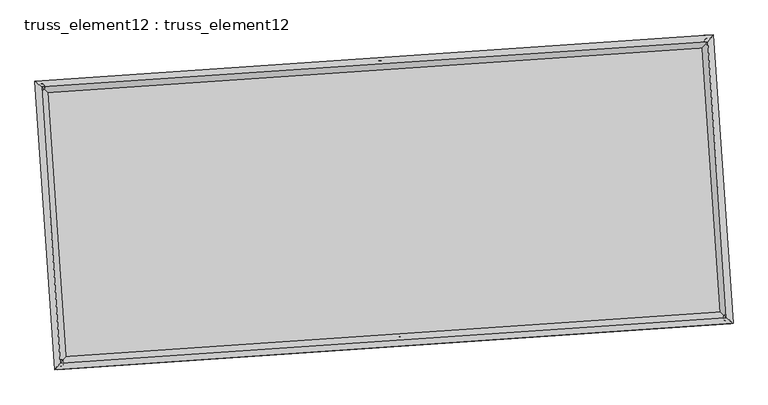
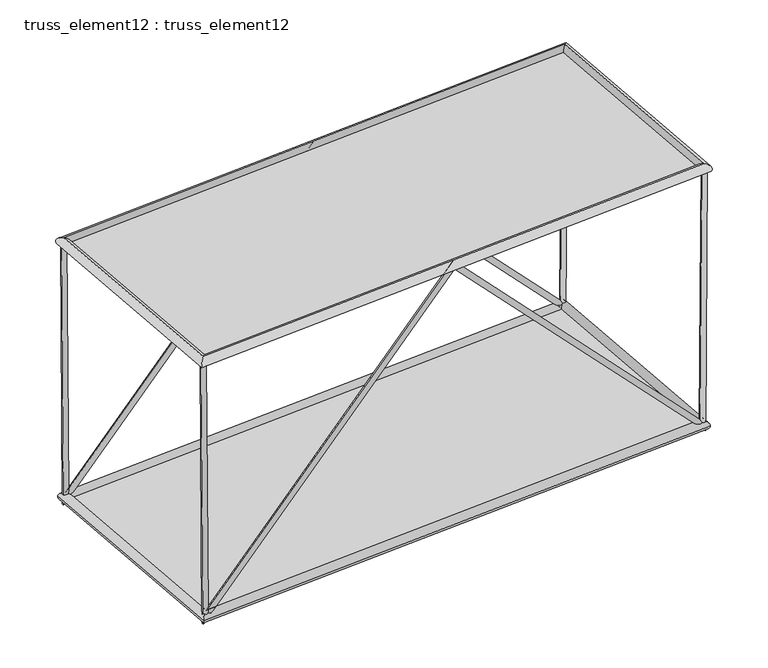
"""IFC4 building model written with IfcOpenShell, lengths in millimetres: plate geometry, truss_element12 : truss_element12."""

from ifc_helpers import new_model, si_unit, frame, origin, origin_with_axes, place, context, project, spatial, polyline, circle_curve, ellipse_curve, outline, extrude, source, transform, mapped, element, save
from ifc_brep_helpers import plane_surface, cylinder_surface, advanced_brep


def truss_element12_truss_element12_8b6da639(model_context):
    return source(origin(), model_context, "Body", "SolidModel", [
        advanced_brep(
        [(-3700.3653821, 2273.8085663, 5000.2282154), (-3799.4662365, 2260.4474806, 4999.5196659), (-3665.8139539, 2276.1644968, 123.2875786), (-3763.1729289, 2262.9221833, -123.2875786), (1064.0023703, 2598.6726923, 5071.9949185), (1064.4463477, 2592.0991902, 4927.7489333), (5793.2665802, 2921.1432411, 123.2835929), (5891.4943968, 2921.2372474, -123.2835929), (5828.3659378, 2923.5365329, 5000.2298034), (5928.3631169, 2923.7511852, 4999.5100189)],
        [
            (0, 1, circle_curve(frame((-3749.9158093, 2267.1280234, 4999.8739406), z_axis=(-0.007084473580338079, -0.0004830633228379881, 0.9999747881241386), x_axis=(-0.13361091131504388, 0.9910337559845098, -0.00046784270723809073)), 50.0)),
            (1, 0, circle_curve(frame((-3749.9158093, 2267.1280234, 4999.8739406), z_axis=(-0.007084473580338079, -0.0004830633228379881, 0.9999747881241386), x_axis=(-0.13361091131504388, 0.9910337559845098, -0.00046784270723809073)), 50.0)),
            (0, 2),
            (2, 3, ellipse_curve(frame((-3714.4934414, 2269.54334, 0.0), z_axis=(-0.9270962013206413, -0.06321516574545871, 0.3694542953013412), x_axis=(0.3685984160306923, 0.025133324815376896, 0.9292489029766943)), 132.9633385, 50.0)),
            (3, 1),
            (3, 2, ellipse_curve(frame((-3714.4934414, 2269.54334, 0.0), z_axis=(-0.9270962013206413, -0.06321516574545871, 0.3694542953013412), x_axis=(0.3685984160306923, 0.025133324815376896, 0.9292489029766943)), 132.9633385, 50.0)),
            (2, 4),
            (4, 5, ellipse_curve(frame((1064.224359, 2595.3859413, 4999.8719259), z_axis=(-0.9976833956449117, -0.06802823819938442, 2.935858576566568e-05), x_axis=(-2.929057355045047e-05, -1.9972128665769184e-06, -0.9999999995690367)), 72.2800399, 50.0)),
            (5, 3),
            (5, 4, ellipse_curve(frame((1064.224359, 2595.3859413, 4999.8719259), z_axis=(-0.9976833956449117, -0.06802823819938442, 2.935858576566568e-05), x_axis=(-2.929057355045047e-05, -1.9972128665769184e-06, -0.9999999995690367)), 72.2800399, 50.0)),
            (4, 6),
            (6, 7, ellipse_curve(frame((5842.3804885, 2921.1902443, 0.0), z_axis=(-0.9271277711546797, -0.0632173183724334, -0.3693746967667848), x_axis=(-0.3685190018944136, -0.02512790986730541, 0.9292805461153513)), 132.9545126, 50.0)),
            (7, 5),
            (7, 6, ellipse_curve(frame((5842.3804885, 2921.1902443, 0.0), z_axis=(-0.9271277711546797, -0.0632173183724334, -0.3693746967667848), x_axis=(-0.3685190018944136, -0.02512790986730541, 0.9292805461153513)), 132.9545126, 50.0)),
            (8, 9, circle_curve(frame((5878.3645274, 2923.6438591, 4999.8699112), z_axis=(0.007196807775672843, 0.0004907229645955706, 0.9999739822359441), x_axis=(-0.002149999800475158, 0.9999975758109794, -0.00047526100493728435)), 50.0)),
            (9, 8, circle_curve(frame((5878.3645274, 2923.6438591, 4999.8699112), z_axis=(0.007196807775672843, 0.0004907229645955706, 0.9999739822359441), x_axis=(-0.002149999800475158, 0.9999975758109794, -0.00047526100493728435)), 50.0)),
            (6, 8),
            (9, 7),
        ],
        [
            plane_surface(frame((-3749.9158093, 2317.1280176, 4999.8980944), z_axis=(-0.0070844735803373745, -0.00048306332284137114, 0.9999747881241386), x_axis=(0.9999749048021603, -3.422335232095009e-06, 0.007084472753714267))),
            cylinder_surface(frame((-3749.9158093, 2267.1280234, 4999.8739406), z_axis=(-0.007084473580338079, -0.0004830633228379881, 0.9999747881241386), x_axis=(-0.13361091131504388, 0.9910337559845098, -0.00046784270723809073)), 50.0),
            cylinder_surface(frame((-3714.4934414, 2269.54334, 0.0), z_axis=(-0.690172538563737, -0.0470602418132238, -0.7221130109982568), x_axis=(-0.020414395916308354, 0.9987521960693102, -0.04557744273324799)), 50.0),
            cylinder_surface(frame((1064.224359, 2595.3859413, 4999.8719259), z_axis=(-0.6901302351654778, -0.04705735730530667, 0.7221536288310701), x_axis=(-0.1153491321235071, 0.9922789572880589, -0.04557464911193756)), 50.0),
            plane_surface(frame((5878.3645274, 2873.6438651, 4999.894448), z_axis=(0.007196807775673034, 0.0004907229645977637, 0.999973982235944), x_axis=(0.9999741026435836, -3.531730309092038e-06, -0.007196806909099957))),
            cylinder_surface(frame((5842.3804885, 2921.1902443, 0.0), z_axis=(-0.007196807775672843, -0.0004907229645955706, -0.9999739822359441), x_axis=(-0.002149999800475158, 0.9999975758109794, -0.00047526100493728435)), 50.0),
        ],
        [
            (0, [[1, 2]]),
            (1, [[-1, 3, 4, 5]]),
            (1, [[-2, -5, 6, -3]]),
            (2, [[-4, 7, 8, 9]]),
            (2, [[-6, -9, 10, -7]]),
            (3, [[-8, 11, 12, 13]]),
            (3, [[-10, -13, 14, -11]]),
            (4, [[15, 16]]),
            (5, [[-12, 17, -16, 18]]),
            (5, [[-14, -18, -15, -17]]),
        ],
    ),
        advanced_brep(
        [(-3428.2524292, -1716.925018, 5000.2282154), (-3527.3532836, -1730.2861037, 4999.5196659), (-3393.701001, -1714.5690875, 123.2875786), (-3491.059976, -1727.811401, -123.2875786), (1336.1153232, -1392.060892, 5071.9949185), (1336.5593007, -1398.6343941, 4927.7489333), (6065.3795331, -1069.5903432, 123.2835929), (6163.6073497, -1069.4963369, -123.2835929), (6100.4788907, -1067.1970514, 5000.2298034), (6200.4760699, -1066.9823991, 4999.5100189)],
        [
            (0, 1, circle_curve(frame((-3477.8028564, -1723.6055609, 4999.8739406), z_axis=(-0.00708447358033807, -0.0004830633228380067, 0.9999747881241386), x_axis=(-0.13361091131504368, 0.9910337559845098, -0.00046784270723806986)), 50.0)),
            (1, 0, circle_curve(frame((-3477.8028564, -1723.6055609, 4999.8739406), z_axis=(-0.00708447358033807, -0.0004830633228380067, 0.9999747881241386), x_axis=(-0.13361091131504368, 0.9910337559845098, -0.00046784270723806986)), 50.0)),
            (0, 2),
            (2, 3, ellipse_curve(frame((-3442.3804885, -1721.1902443, 0.0), z_axis=(-0.9270962013206415, -0.06321516574545867, 0.3694542953013411), x_axis=(0.3685984160306922, 0.025133324815376848, 0.9292489029766942)), 132.9633385, 50.0)),
            (3, 1),
            (3, 2, ellipse_curve(frame((-3442.3804885, -1721.1902443, 0.0), z_axis=(-0.9270962013206415, -0.06321516574545867, 0.3694542953013411), x_axis=(0.3685984160306922, 0.025133324815376848, 0.9292489029766942)), 132.9633385, 50.0)),
            (2, 4),
            (4, 5, ellipse_curve(frame((1336.3373119, -1395.347643, 4999.8719259), z_axis=(-0.9976833956449116, -0.06802823819938435, 2.9358585765665695e-05), x_axis=(-2.92905735506042e-05, -1.997212866576918e-06, -0.9999999995690367)), 72.2800399, 50.0)),
            (5, 3),
            (5, 4, ellipse_curve(frame((1336.3373119, -1395.347643, 4999.8719259), z_axis=(-0.9976833956449116, -0.06802823819938435, 2.9358585765665695e-05), x_axis=(-2.92905735506042e-05, -1.997212866576918e-06, -0.9999999995690367)), 72.2800399, 50.0)),
            (4, 6),
            (6, 7, ellipse_curve(frame((6114.4934414, -1069.54334, 0.0), z_axis=(-0.9271277711546799, -0.06321731837243338, -0.36937469676678447), x_axis=(-0.3685190018944132, -0.02512790986730538, 0.9292805461153515)), 132.9545126, 50.0)),
            (7, 5),
            (7, 6, ellipse_curve(frame((6114.4934414, -1069.54334, 0.0), z_axis=(-0.9271277711546799, -0.06321731837243338, -0.36937469676678447), x_axis=(-0.3685190018944132, -0.02512790986730538, 0.9292805461153515)), 132.9545126, 50.0)),
            (8, 9, circle_curve(frame((6150.4774803, -1067.0897252, 4999.8699112), z_axis=(0.007196807775673056, 0.0004907229645955708, 0.9999739822359441), x_axis=(-0.0021499998004751303, 0.9999975758109794, -0.00047526100493728435)), 50.0)),
            (9, 8, circle_curve(frame((6150.4774803, -1067.0897252, 4999.8699112), z_axis=(0.007196807775673056, 0.0004907229645955708, 0.9999739822359441), x_axis=(-0.0021499998004751303, 0.9999975758109794, -0.00047526100493728435)), 50.0)),
            (6, 8),
            (9, 7),
        ],
        [
            plane_surface(frame((-3477.8028564, -1673.6055667, 4999.8980944), z_axis=(-0.007084473580337374, -0.00048306332284136583, 0.9999747881241385), x_axis=(0.9999749048021603, -3.422335232095009e-06, 0.007084472753714267))),
            cylinder_surface(frame((-3477.8028564, -1723.6055609, 4999.8739406), z_axis=(-0.00708447358033807, -0.0004830633228380067, 0.9999747881241386), x_axis=(-0.13361091131504368, 0.9910337559845098, -0.00046784270723806986)), 50.0),
            cylinder_surface(frame((-3442.3804885, -1721.1902443, 0.0), z_axis=(-0.6901725385637364, -0.047060241813223706, -0.7221130109982571), x_axis=(-0.020414395916308312, 0.9987521960693102, -0.045577442733247896)), 50.0),
            cylinder_surface(frame((1336.3373119, -1395.347643, 4999.8719259), z_axis=(-0.6901302351654776, -0.047057357305306635, 0.7221536288310705), x_axis=(-0.11534913212350704, 0.9922789572880589, -0.04557464911193748)), 50.0),
            plane_surface(frame((6150.4774803, -1117.0897192, 4999.894448), z_axis=(0.007196807775673035, 0.0004907229645977578, 0.999973982235944), x_axis=(0.9999741026435836, -3.5317303099802163e-06, -0.007196806909099957))),
            cylinder_surface(frame((6114.4934414, -1069.54334, 0.0), z_axis=(-0.007196807775673056, -0.0004907229645955708, -0.9999739822359441), x_axis=(-0.0021499998004751303, 0.9999975758109794, -0.00047526100493728435)), 50.0),
        ],
        [
            (0, [[1, 2]]),
            (1, [[-1, 3, 4, 5]]),
            (1, [[-2, -5, 6, -3]]),
            (2, [[-4, 7, 8, 9]]),
            (2, [[-6, -9, 10, -7]]),
            (3, [[-8, 11, 12, 13]]),
            (3, [[-10, -13, 14, -11]]),
            (4, [[15, 16]]),
            (5, [[-12, 17, -16, 18]]),
            (5, [[-14, -18, -15, -17]]),
        ],
    ),
        advanced_brep(
        [(-3477.8039198, -1723.6067394, 4909.8739406), (-3477.801793, -1723.6043823, 5089.8739406), (-3749.9145958, 2267.1270001, 5089.8739406), (-3749.9170228, 2267.1290467, 4909.8739406), (5878.363539, 2923.6426856, 5089.8699112), (5878.3655158, 2923.6450325, 4909.8699112), (6150.4763418, -1067.0886968, 5089.8699112), (6150.4786188, -1067.0907536, 4909.8699112)],
        [
            (0, 1, ellipse_curve(frame((-3477.8028564, -1723.6055609, 4999.8739406), z_axis=(-0.7535719234053952, 0.6573654662780863, 2.952390620446819e-07), x_axis=(-0.6573654662780205, -0.7535719234054525, 2.95239062044708e-07)), 127.2792206, 90.0)),
            (1, 2),
            (2, 3, ellipse_curve(frame((-3749.9158093, 2267.1280234, 4999.8739406), z_axis=(-0.6573654662780207, -0.7535719234054526, 2.952390620447316e-07), x_axis=(0.7535719234053954, -0.6573654662780862, -2.9523906204470547e-07)), 127.2792206, 90.0)),
            (3, 0),
            (1, 0, ellipse_curve(frame((-3477.8028564, -1723.6055609, 4999.8739406), z_axis=(-0.7535719234053952, 0.6573654662780863, 2.952390620446819e-07), x_axis=(-0.6573654662780205, -0.7535719234054525, 2.95239062044708e-07)), 127.2792206, 90.0)),
            (3, 2, ellipse_curve(frame((-3749.9158093, 2267.1280234, 4999.8739406), z_axis=(-0.6573654662780207, -0.7535719234054526, 2.952390620447316e-07), x_axis=(0.7535719234053954, -0.6573654662780862, -2.9523906204470547e-07)), 127.2792206, 90.0)),
            (2, 4),
            (4, 5, ellipse_curve(frame((5878.3645274, 2923.6438591, 4999.8699112), z_axis=(-0.7535719234053952, 0.6573654662780863, 2.952390620447292e-07), x_axis=(-0.6573654662780208, -0.7535719234054525, 2.952390620447079e-07)), 127.2792206, 90.0)),
            (5, 3),
            (5, 4, ellipse_curve(frame((5878.3645274, 2923.6438591, 4999.8699112), z_axis=(-0.7535719234053952, 0.6573654662780863, 2.952390620447292e-07), x_axis=(-0.6573654662780208, -0.7535719234054525, 2.952390620447079e-07)), 127.2792206, 90.0)),
            (4, 6),
            (6, 7, ellipse_curve(frame((6150.4774803, -1067.0897252, 4999.8699112), z_axis=(0.6573654662780207, 0.7535719234054526, -2.9523906204468435e-07), x_axis=(-0.7535719234053954, 0.6573654662780862, 2.952390620447057e-07)), 127.2792206, 90.0)),
            (7, 5),
            (7, 6, ellipse_curve(frame((6150.4774803, -1067.0897252, 4999.8699112), z_axis=(0.6573654662780207, 0.7535719234054526, -2.9523906204468435e-07), x_axis=(-0.7535719234053954, 0.6573654662780862, 2.952390620447057e-07)), 127.2792206, 90.0)),
            (6, 1),
            (0, 7),
        ],
        [
            cylinder_surface(frame((-3477.8028564, -1723.6055609, 4999.8739406), z_axis=(0.06802823822870009, -0.9976833960748767, 0.0), x_axis=(-0.9976833959946901, -0.06802823822323248, 1.2678541203017778e-05)), 90.0),
            cylinder_surface(frame((-3749.9158093, 2267.1280234, 4999.8739406), z_axis=(-0.9976833960747897, -0.06802823822869289, 4.175310856859526e-07), x_axis=(-0.0680282382184779, 0.9976833960002329, 1.2261010117363229e-05)), 90.0),
            cylinder_surface(frame((5878.3645274, 2923.6438591, 4999.8699112), z_axis=(-0.06802823822870009, 0.9976833960748767, 0.0), x_axis=(0.9976833960049052, 0.06802823822392899, 1.1843479031708684e-05)), 90.0),
            cylinder_surface(frame((6150.4774803, -1067.0897252, 4999.8699112), z_axis=(0.9976833960747897, 0.06802823822869286, -4.175310856859193e-07), x_axis=(0.06802823822869286, -0.9976833959995364, 1.226101011736324e-05)), 90.0),
        ],
        [
            (0, [[1, 2, 3, 4]]),
            (0, [[5, -4, 6, -2]]),
            (1, [[-3, 7, 8, 9]]),
            (1, [[-6, -9, 10, -7]]),
            (2, [[-8, 11, 12, 13]]),
            (2, [[-10, -13, 14, -11]]),
            (3, [[-12, 15, -1, 16]]),
            (3, [[-14, -16, -5, -15]]),
        ],
    ),
        advanced_brep(
        [(-3358.7115243, -1625.2761972, 0.0), (-3526.0494527, -1817.1042913, 0.0), (-3810.4074885, 2353.2123043, 0.0), (-3618.5793943, 2185.8743758, 0.0), (5926.0494527, 3017.1042913, 0.0), (5758.7115243, 2825.2761972, 0.0), (6210.4074885, -1153.2123043, 0.0), (6018.5793943, -985.8743758, 0.0)],
        [
            (0, 1, ellipse_curve(frame((-3442.3804885, -1721.1902443, 0.0), z_axis=(-0.7535719234054589, 0.6573654662780799, 0.0), x_axis=(-0.6573654662780799, -0.7535719234054586, 0.0)), 127.2792206, 90.0)),
            (1, 2),
            (2, 3, ellipse_curve(frame((-3714.4934414, 2269.54334, 0.0), z_axis=(-0.6573654662780798, -0.7535719234054586, 0.0), x_axis=(0.7535719234054585, -0.6573654662780801, 0.0)), 127.2792206, 90.0)),
            (3, 0),
            (1, 0, ellipse_curve(frame((-3442.3804885, -1721.1902443, 0.0), z_axis=(-0.7535719234054589, 0.6573654662780799, 0.0), x_axis=(-0.6573654662780799, -0.7535719234054586, 0.0)), 127.2792206, 90.0)),
            (3, 2, ellipse_curve(frame((-3714.4934414, 2269.54334, 0.0), z_axis=(-0.6573654662780798, -0.7535719234054586, 0.0), x_axis=(0.7535719234054585, -0.6573654662780801, 0.0)), 127.2792206, 90.0)),
            (2, 4),
            (4, 5, ellipse_curve(frame((5842.3804885, 2921.1902443, 0.0), z_axis=(-0.7535719234054589, 0.6573654662780799, 0.0), x_axis=(-0.6573654662780795, -0.753571923405459, 0.0)), 127.2792206, 90.0)),
            (5, 3),
            (5, 4, ellipse_curve(frame((5842.3804885, 2921.1902443, 0.0), z_axis=(-0.7535719234054589, 0.6573654662780799, 0.0), x_axis=(-0.6573654662780795, -0.753571923405459, 0.0)), 127.2792206, 90.0)),
            (4, 6),
            (6, 7, ellipse_curve(frame((6114.4934414, -1069.54334, 0.0), z_axis=(0.6573654662780798, 0.7535719234054586, 0.0), x_axis=(-0.7535719234054585, 0.6573654662780801, 0.0)), 127.2792206, 90.0)),
            (7, 5),
            (7, 6, ellipse_curve(frame((6114.4934414, -1069.54334, 0.0), z_axis=(0.6573654662780798, 0.7535719234054586, 0.0), x_axis=(-0.7535719234054585, 0.6573654662780801, 0.0)), 127.2792206, 90.0)),
            (6, 1),
            (0, 7),
        ],
        [
            cylinder_surface(frame((-3442.3804885, -1721.1902443, 0.0), z_axis=(0.068028238228703, -0.9976833960748764, 0.0), x_axis=(-0.9976833960748764, -0.068028238228703, 0.0)), 90.0),
            cylinder_surface(frame((-3714.4934414, 2269.54334, 0.0), z_axis=(-0.9976833960748765, -0.06802823822870202, 0.0), x_axis=(-0.06802823822870202, 0.9976833960748765, 0.0)), 90.0),
            cylinder_surface(frame((5842.3804885, 2921.1902443, 0.0), z_axis=(-0.06802823822870302, 0.9976833960748764, 0.0), x_axis=(0.9976833960748764, 0.06802823822870302, 0.0)), 90.0),
            cylinder_surface(frame((6114.4934414, -1069.54334, 0.0), z_axis=(0.9976833960748765, 0.06802823822870203, 0.0), x_axis=(0.06802823822870203, -0.9976833960748765, 0.0)), 90.0),
        ],
        [
            (0, [[1, 2, 3, 4]]),
            (0, [[5, -4, 6, -2]]),
            (1, [[-3, 7, 8, 9]]),
            (1, [[-6, -9, 10, -7]]),
            (2, [[-8, 11, 12, 13]]),
            (2, [[-10, -13, 14, -11]]),
            (3, [[-12, 15, -1, 16]]),
            (3, [[-14, -16, -5, -15]]),
        ],
    ),
        extrude(outline(polyline([(-3442.3804885, -1721.1902443), (-3714.4934414, 2269.54334), (5842.3804885, 2921.1902443), (6114.4934414, -1069.54334), (-3442.3804885, -1721.1902443)])), origin_with_axes(), (0.0, 0.0, 1.0), 20.0),
        extrude(outline(polyline([(-2000.0, 4825.3185202), (2000.0, 4825.3185202), (2000.0, -4825.3185202), (-2000.0, -4825.3185202), (-2000.0, 4825.3185202)])), frame((1200.2808355, 600.0191491, 4999.8719259), z_axis=(4.165638315339748e-07, 2.840390416493192e-08, 0.9999999999999128), x_axis=(-0.06802823822870314, 0.9976833960748764, 0.0)), (0.0, 0.0, 1.0), 20.0),
    ])


if __name__ == "__main__":
    model = new_model("IFC4")
    model_context = context("Model", 3, world=origin())
    ifc_project = project(units=[si_unit("LENGTHUNIT", "METRE", prefix="MILLI")], contexts=[model_context])
    site = spatial("IfcSite", under=ifc_project)
    building = spatial("IfcBuilding", under=site)
    placement = place(None, origin())
    truss_element12_truss_element12_shape = truss_element12_truss_element12_8b6da639(model_context)
    element("IfcPlate", 1, ObjectType="truss_element12 : truss_element12", at=placement, inside=building, context=model_context, shape_type="MappedRepresentation", body=[
        mapped(truss_element12_truss_element12_shape, transform((0.0, 0.0, 0.0), x_axis=(1.0, 0.0, 0.0), y_axis=(0.0, 1.0, 0.0), z_axis=(0.0, 0.0, 1.0))),
    ])
    save(model, "model.ifc")

# Revit data of these elements
# Type "truss_element12 : truss_element12"
#   steellbar1 = 90 mm
#   steelbar2 = 50 mm
#   offset1 = 5000 mm
#   M = Default Roof
# Element 1 (IfcPlate, "truss_element12 : truss_element12")
#   Materials on its faces: "Default Roof"
# Materials
#   "Default Roof": class "Miscellaneous", colour RGB 0 127 0, transparency 0, Comments = "Rendering appearance not upgraded Rendering appearance not upgraded ", Cost = 0
